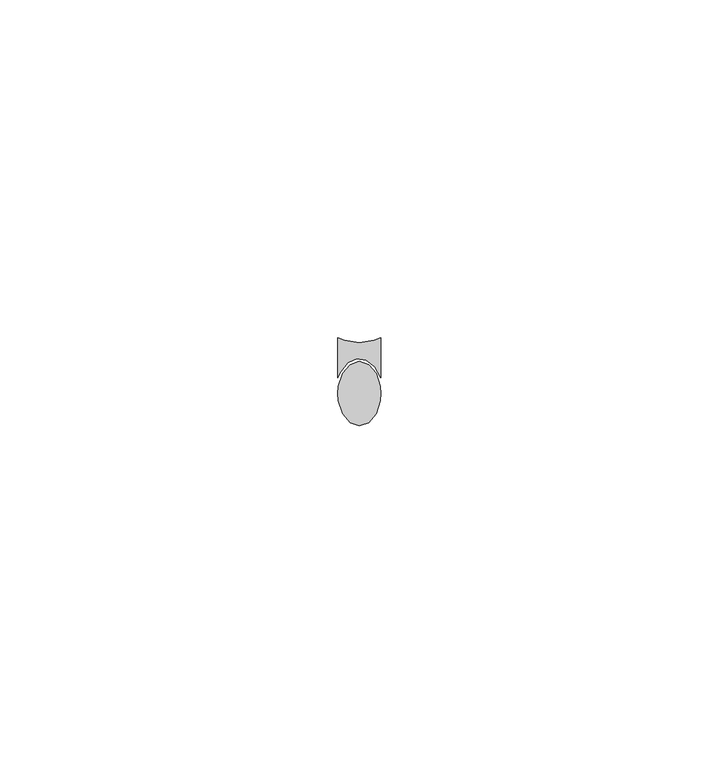
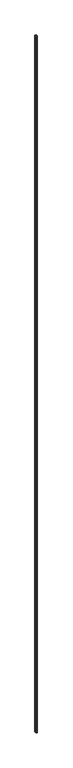
"""IFC4 building model written with IfcOpenShell, lengths in millimetres: proxy geometry, Generic Models 11:Generic Models 1:306267:Generic Models 1:306267 : Generic Models 11:Generic Models 1:306267:300405:Generic Models 1:306267:Generic Models 1:306267 : Generic Models 11:Generic Models 1:306267:300405 : Generic Models 11:Generic Models 1:306267:Generic Models 1:306267 : Generic Models 11:Generic Models 1:306267:300405:12 : Generic Models 11:Generic Models 1:306267:Generic Models 1:306267 : Generic Models 11:Generic Models 1:306267:300405:Generic Models 1:306267:Generic Models 1:306267 : Generic Models 11:Generic Models 1:306267:300405 : Generic Models 11:Generic Models 1:306267:Generic Models 1:306267 : Generic Models 11:Generic Models 1:306267:300405:300182."""

from ifc_helpers import new_model, si_unit, origin, origin_with_axes, place, context, project, spatial, polyline, outline, extrude, source, transform, mapped, element, save


def generic_models_7cfbd7db(model_context):
    return source(origin(), model_context, "Body", "SweptSolid", [
        extrude(outline(polyline([(592757.2216431, -579036.3403513), (592758.5992239, -579035.8687155), (592759.9768048, -579036.3403513), (592761.0815389, -579037.6618453), (592761.6946201, -579039.5714595), (592761.7742239, -579040.6312155), (592761.6946201, -579041.6909714), (592761.0815389, -579043.6005857), (592759.9768048, -579044.9220797), (592758.5992239, -579045.3937155), (592757.2216431, -579044.9220797), (592756.116909, -579043.6005857), (592755.5038278, -579041.6909714), (592755.4242239, -579040.6312155), (592755.5038278, -579039.5714595), (592756.116909, -579037.6618453), (592757.2216431, -579036.3403513)])), origin_with_axes(), (0.0, 0.0, 1.0), 3695.7),
        extrude(outline(polyline([(592760.8084607, -579032.7769044), (592761.7742239, -579032.3994958), (592761.7742239, -579038.2675879), (592760.8914351, -579036.6743712), (592759.650051, -579035.7001662), (592758.2442747, -579035.4973783), (592756.894027, -579036.0977318), (592755.8105415, -579037.4073069), (592755.4242239, -579038.2675879), (592755.4242239, -579032.3994958), (592756.3899872, -579032.7769044), (592758.5992239, -579033.0905905), (592760.8084607, -579032.7769044)])), origin_with_axes(), (0.0, 0.0, 1.0), 3695.7),
    ])


if __name__ == "__main__":
    model = new_model("IFC4")
    model_context = context("Model", 3, world=origin())
    ifc_project = project(units=[si_unit("LENGTHUNIT", "METRE", prefix="MILLI")], contexts=[model_context])
    site = spatial("IfcSite", under=ifc_project)
    building = spatial("IfcBuilding", under=site)
    placement = place(None, origin())
    generic_models_shape = generic_models_7cfbd7db(model_context)
    element("IfcBuildingElementProxy", 1, Name="Generic Models 11:Generic Models 1:306267:Generic Models 1:306267 : Generic Models 11:Generic Models 1:306267:300405:Generic Models 1:306267:Generic Models 1:306267 : Generic Models 11:Generic Models 1:306267:300405 : Generic Models 11:Generic Models 1:306267:Generic Models 1:306267 : Generic Models 11:Generic Models 1:306267:300405:12 : Generic Models 11:Generic Models 1:306267:Generic Models 1:306267 : Generic Models 11:Generic Models 1:306267:300405:Generic Models 1:306267:Generic Models 1:306267 : Generic Models 11:Generic Models 1:306267:300405 : Generic Models 11:Generic Models 1:306267:Generic Models 1:306267 : Generic Models 11:Generic Models 1:306267:300405:300182", ObjectType="Generic Models 11:Generic Models 1:306267:Generic Models 1:306267 : Generic Models 11:Generic Models 1:306267:300405:Generic Models 1:306267:Generic Models 1:306267 : Generic Models 11:Generic Models 1:306267:300405 : Generic Models 11:Generic Models 1:306267:Generic Models 1:306267 : Generic Models 11:Generic Models 1:306267:300405:12 : Generic Models 11:Generic Models 1:306267:Generic Models 1:306267 : Generic Models 11:Generic Models 1:306267:300405:Generic Models 1:306267:Generic Models 1:306267 : Generic Models 11:Generic Models 1:306267:300405 : Generic Models 11:Generic Models 1:306267:Generic Models 1:306267 : Generic Models 11:Generic Models 1:306267:300405:300182", at=placement, inside=building, context=model_context, shape_type="MappedRepresentation", body=[
        mapped(generic_models_shape, transform((0.0, 0.0, 0.0), x_axis=(1.0, 0.0, 0.0), y_axis=(0.0, 1.0, 0.0), z_axis=(0.0, 0.0, 1.0))),
    ])
    save(model, "model.ifc")

# Revit data of these elements
# Type "Generic Models 11:Generic Models 1:306267:Generic Models 1:306267 : Generic Models 11:Generic Models 1:306267:300405:Generic Models 1:306267:Generic Models 1:306267 : Generic Models 11:Generic Models 1:306267:300405 : Generic Models 11:Generic Models 1:306267:Generic Models 1:306267 : Generic Models 11:Generic Models 1:306267:300405:12 : Generic Models 11:Generic Models 1:306267:Generic Models 1:306267 : Generic Models 11:Generic Models 1:306267:300405:Generic Models 1:306267:Generic Models 1:306267 : Generic Models 11:Generic Models 1:306267:300405 : Generic Models 11:Generic Models 1:306267:Generic Models 1:306267 : Generic Models 11:Generic Models 1:306267:300405:300182"
#   NameOverride = "Generic Models 11:Generic Models 1:306267:Generic Models 1:306267 : Generic Models 11:Generic Models 1:306267:300405:Generic Models 1:306267:Generic Models 1:306267 : Generic Models 11:Generic Models 1:306267:300405 : Generic Models 11:Generic Models 1:306267:Generic Models 1:306267 : Generic Models 11:Generic Models 1:306267:300405:300182"
#   ObjectTypeOverride = "Generic Models 1:306267:Generic Models 1:306267 : Generic Models 11:Generic Models 1:306267:300405 : Generic Models 11:Generic Models 1:306267:Generic Models 1:306267 : Generic Models 11:Generic Models 1:306267:300405"
#   Reference = "Generic Models 1"
#   Tag = "300182"
# Element 1 (IfcBuildingElementProxy, "Generic Models 11:Generic Models 1:306267:Generic Models 1:306267 : Generic Models 11:Generic Models 1:306267:300405:Generic Models 1:306267:Generic Models 1:306267 : Generic Models 11:Generic Models 1:306267:300405 : Generic Models 11:Generic Models 1:306267:Generic Models 1:306267 : Generic Models 11:Generic Models 1:306267:300405:12 : Generic Models 11:Generic Models 1:306267:Generic Models 1:306267 : Generic Models 11:Generic Models 1:306267:300405:Generic Models 1:306267:Generic Models 1:306267 : Generic Models 11:Generic Models 1:306267:300405 : Generic Models 11:Generic Models 1:306267:Generic Models 1:306267 : Generic Models 11:Generic Models 1:306267:300405:300182")
#   Materials on its faces: "SEALANT & BACKER ROD"
# Materials
#   "SEALANT & BACKER ROD": class "Unassigned", colour RGB 120 120 120, transparency 0, Cost = 0
